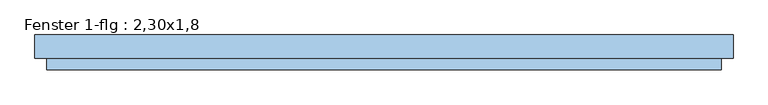
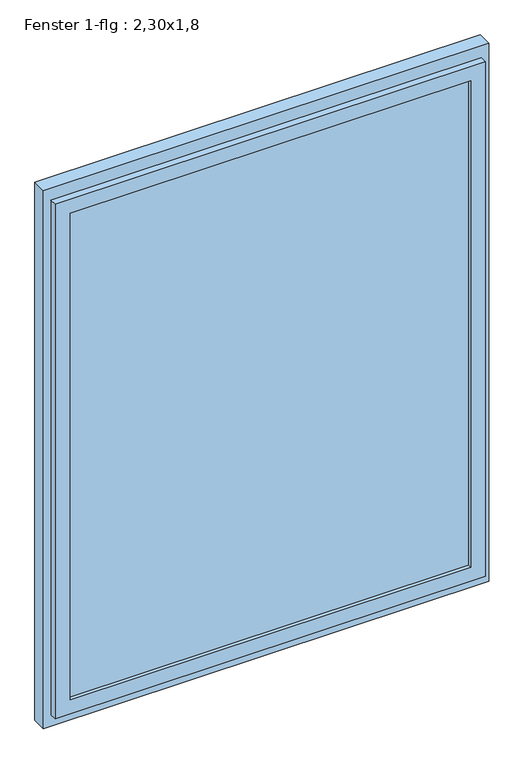
"""IFC4 building model written with IfcOpenShell, lengths in millimetres: window geometry, Fenster 1-flg : 2,30x1,8."""

from ifc_helpers import new_model, si_unit, frame, origin, place, context, project, spatial, polyline, outline, extrude, faceted_brep, source, transform, mapped, element, save


def fenster_1_flg_2_30x1_8_8c7a4049(model_context):
    return source(origin(), model_context, "Body", "SolidModel", [
        extrude(outline(polyline([(3300.0, 900.0), (3300.0, -900.0), (1000.0, -900.0), (1000.0, 900.0), (3300.0, 900.0)]), holes=[polyline([(3220.0, 840.0), (1080.0, 840.0), (1080.0, -840.0), (3220.0, -840.0), (3220.0, 840.0)])]), frame((0.0, -30.0, 0.0), z_axis=(0.0, 1.0, 0.0), x_axis=(0.0, 0.0, 1.0)), (0.0, 0.0, 1.0), 60.0),
        faceted_brep([(870.0, -30.0, 3250.0), (870.0, -60.0, 3250.0), (870.0, -60.0, 1050.0), (870.0, -30.0, 1050.0), (-870.0, -60.0, 3250.0), (-870.0, -60.0, 1050.0), (810.0, -60.0, 1110.0), (-810.0, -60.0, 1110.0), (-810.0, -60.0, 3190.0), (810.0, -60.0, 3190.0), (-870.0, -30.0, 1050.0), (-870.0, -30.0, 3250.0), (840.0, -30.0, 3220.0), (-840.0, -30.0, 3220.0), (-840.0, -30.0, 1080.0), (840.0, -30.0, 1080.0), (840.0, 0.0, 3220.0), (840.0, 0.0, 1080.0), (-840.0, 0.0, 1080.0), (-840.0, 0.0, 3220.0), (810.0, 0.0, 3190.0), (-810.0, 0.0, 3190.0), (-810.0, 0.0, 1110.0), (810.0, 0.0, 1110.0)], [[[0, 1, 2, 3]], [[1, 4, 5, 2], [6, 7, 8, 9]], [[3, 2, 5, 10]], [[3, 10, 11, 0], [12, 13, 14, 15]], [[16, 12, 15, 17]], [[17, 15, 14, 18]], [[17, 18, 19, 16], [20, 21, 22, 23]], [[9, 20, 23, 6]], [[6, 23, 22, 7]], [[10, 5, 4, 11]], [[18, 14, 13, 19]], [[7, 22, 21, 8]], [[11, 4, 1, 0]], [[19, 13, 12, 16]], [[8, 21, 20, 9]]]),
        extrude(outline(polyline([(810.0, -45.0), (-810.0, -45.0), (-810.0, -15.0), (810.0, -15.0), (810.0, -45.0)])), frame((0.0, 0.0, 1110.0), z_axis=(0.0, 0.0, 1.0), x_axis=(1.0, 0.0, 0.0)), (0.0, 0.0, 1.0), 2080.0),
    ])


if __name__ == "__main__":
    model = new_model("IFC4")
    model_context = context("Model", 3, world=origin())
    ifc_project = project(units=[si_unit("LENGTHUNIT", "METRE", prefix="MILLI")], contexts=[model_context])
    site = spatial("IfcSite", under=ifc_project)
    building = spatial("IfcBuilding", under=site)
    placement = place(None, origin())
    fenster_1_flg_2_30x1_8_shape = fenster_1_flg_2_30x1_8_8c7a4049(model_context)
    element("IfcWindow", 1, ObjectType="Fenster 1-flg : 2,30x1,8", at=placement, inside=building, context=model_context, shape_type="MappedRepresentation", body=[
        mapped(fenster_1_flg_2_30x1_8_shape, transform((0.0, 0.0, 0.0), x_axis=(1.0, 0.0, 0.0), y_axis=(0.0, 1.0, 0.0), z_axis=(0.0, 0.0, 1.0))),
    ])
    save(model, "model.ifc")

# Revit data of these elements
# Type "Fenster 1-flg : 2,30x1,8"
#   Type Mark = "71"
#   Operation = "SinglePanel"
#   Keynote = "16.05.01"
#   Visual Light Transmittance = 0.9
#   Solar Heat Gain Coefficient = 0.86
#   Rough Width = 1.800 m
#   Rough Height = 2.300 m
#   Heat Transfer Coefficient (U) = 5.5617 W/(m²·K)
#   Rahmentiefe = 0.060 m
#   Rahmenhöhe - unten = 0.080 m
#   Rahmenhöhe - oben = 0.080 m
#   Rahmenbreite = 0.060 m
#   Height = 2.300 m
#   Tiefe Flügel = 0.060 m
#   Flügelbreite = 0.060 m
#   Einbautiefe (von außen) [instance default] = 0.100 m
#   Width = 1.800 m
#   Klappflügel [instance default] = no
#   Kippflügel [instance default] = yes
#   Öffnungsrichtung in Draufsicht anzeigen [instance default] = no
#   Drehflügel 1 [instance default] = yes
#   Rahmen 1 [instance default] = none
#   Glas [instance default] = none
#   Flügel [instance default] = none
#   Fensterbank Innenseite [instance default] = none
#   Fensterbank Außenseite [instance default] = none
#   Construction Type Id = ""
#   Wall Closure = (empty or 0)
#   Analytic Construction = (empty or 0)
# Element 1 (IfcWindow, "Fenster 1-flg : 2,30x1,8")
#   Einbautiefe (von außen) = 0.120 m
#   Materials on its faces: "Kunststoff - Weiß", "Glas"
# Materials
#   "Kunststoff - Weiß": class "Kunststoff", colour RGB 249 249 249, transparency 0, Cost = 0
#   "Glas": class "Glas", colour RGB 0 0 255, transparency 0.75, Comments = "Render-Darstellung nicht aktualisiert ", Cost = 0
